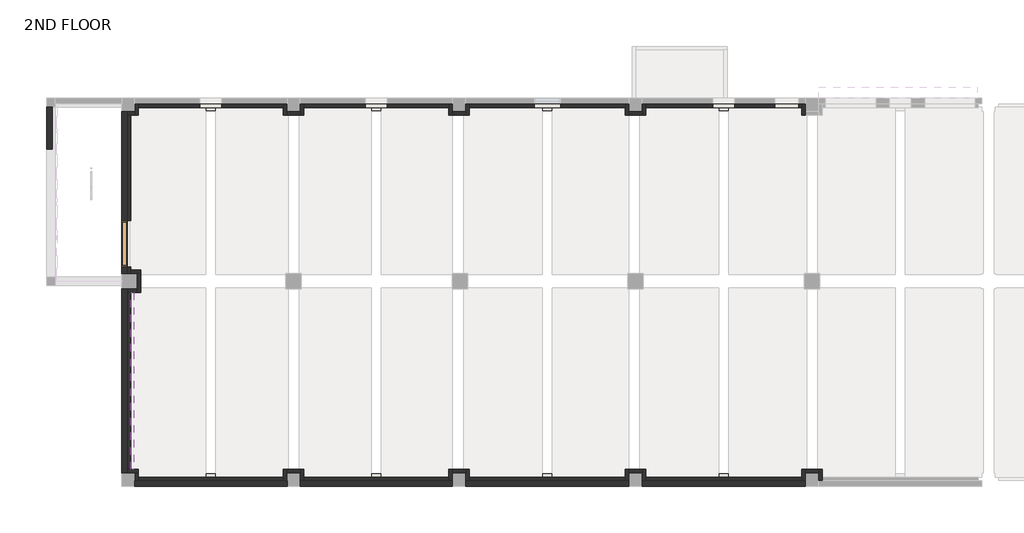
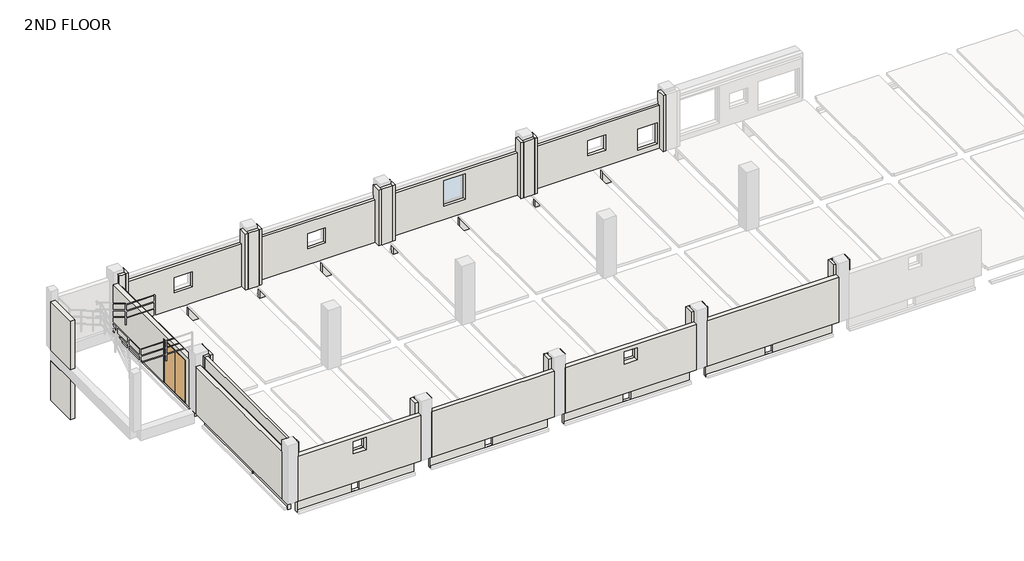
# One storey, part 1 of 7: 60 walls, 1 door.
"""IFC4 building model written with IfcOpenShell, lengths in millimetres."""

import ifcopenshell
import ifcopenshell.guid

model = None  # the IFC model being written
_history = None  # IfcOwnerHistory: only IFC2X3 demands one
_inside = {}  # id of a spatial element -> (the spatial element, [elements in it])
_under = {}  # id of a project, library or spatial element -> (it, [spatial elements below it])
_declared = {}  # id of a project -> (the project, [libraries it declares])
_typed = {}  # id of a type object -> (the type object, [elements of that type])
_made_of = {}  # id of a material, layer set ... -> (it, [elements and type objects made of it])


def new_model(schema):
    """Start an empty IFC model of exactly this schema.

    Asked for "IFC4X3", IfcOpenShell would pick the latest addendum, in which some entities
    have other attributes; the version numbers below select the first issue.
    IFC2X3 requires an IfcOwnerHistory on every rooted entity: one is made here for all.
    """
    global model, _history
    if schema == "IFC4X3":
        model = ifcopenshell.file(schema_version=(4, 3, 0, 0))
    else:
        model = ifcopenshell.file(schema=schema)
    _inside.clear()
    _under.clear()
    _declared.clear()
    _typed.clear()
    _made_of.clear()
    _history = None
    if model.schema == "IFC2X3":
        org = make("IfcOrganization", Name="unknown")
        user = make(
            "IfcPersonAndOrganization",
            ThePerson=make("IfcPerson", FamilyName="unknown"),
            TheOrganization=org,
        )
        app = make(
            "IfcApplication",
            ApplicationDeveloper=org,
            Version="unknown",
            ApplicationFullName="unknown",
            ApplicationIdentifier="unknown",
        )
        _history = make(
            "IfcOwnerHistory",
            OwningUser=user,
            OwningApplication=app,
            ChangeAction="ADDED",
            CreationDate=0,
        )
    return model


def make(cls, **values):
    """One entity of the class cls with the attributes given. An attribute that is None is left unset."""
    return model.create_entity(
        cls, **{name: value for name, value in values.items() if value is not None}
    )


def rooted(cls, **values):
    """An entity with a GlobalId (a new one), such as an element, a storey or a relation."""
    return make(cls, GlobalId=ifcopenshell.guid.new(), OwnerHistory=_history, **values)


def si_unit(unit_type, name, prefix=None):
    """IfcSIUnit, for example si_unit("LENGTHUNIT", "METRE", prefix="MILLI")."""
    return make("IfcSIUnit", UnitType=unit_type, Prefix=prefix, Name=name)


def assignment(units):
    """IfcUnitAssignment: the units of a project."""
    return None if units is None else make("IfcUnitAssignment", Units=units)


def point(xyz):
    """IfcCartesianPoint."""
    return None if xyz is None else make("IfcCartesianPoint", Coordinates=xyz)


def direction(xyz):
    """IfcDirection."""
    return None if xyz is None else make("IfcDirection", DirectionRatios=xyz)


def frame(location, z_axis=None, x_axis=None):
    """IfcAxis2Placement3D, a coordinate frame: its origin and axes. An axis left out is left unset."""
    return make(
        "IfcAxis2Placement3D",
        Location=point(location),
        Axis=direction(z_axis),
        RefDirection=direction(x_axis),
    )


def origin():
    """The frame at (0, 0, 0) with its axes left unset."""
    return frame((0.0, 0.0, 0.0))


def place(relative_to, where):
    """IfcLocalPlacement: puts the frame where relative to a parent placement (None: the world)."""
    return make(
        "IfcLocalPlacement", PlacementRelTo=relative_to, RelativePlacement=where
    )


def context(
    kind, dimensions, precision=None, world=None, true_north=None, identifier=None
):
    """IfcGeometricRepresentationContext, for example the 3D "Model" context."""
    return make(
        "IfcGeometricRepresentationContext",
        ContextIdentifier=identifier,
        ContextType=kind,
        CoordinateSpaceDimension=dimensions,
        Precision=precision,
        WorldCoordinateSystem=world,
        TrueNorth=true_north,
    )


def project(units=None, contexts=None):
    """IfcProject with its units and contexts."""
    return rooted(
        "IfcProject",
        Name="project",
        RepresentationContexts=contexts,
        UnitsInContext=assignment(units),
    )


def spatial(cls, under=None, at=None, **own):
    """A site, building, storey or space (cls), placed at a placement, below another one or the project."""
    s = rooted(cls, ObjectPlacement=at, **own)
    if under is not None:
        _under.setdefault(under.id(), (under, []))[1].append(s)
    return s


def polyline(points):
    """IfcPolyline through the points."""
    return make("IfcPolyline", Points=[point(p) for p in points])


def outline(outer, holes=None, kind="AREA"):
    """IfcArbitraryClosedProfileDef: a profile drawn as a closed curve; with holes, ...WithVoids."""
    if holes is None:
        return make("IfcArbitraryClosedProfileDef", ProfileType=kind, OuterCurve=outer)
    return make(
        "IfcArbitraryProfileDefWithVoids",
        ProfileType=kind,
        OuterCurve=outer,
        InnerCurves=holes,
    )


def extrude(swept, where, along, depth):
    """IfcExtrudedAreaSolid: the profile swept, set in the frame where, extruded along a direction by depth."""
    return make(
        "IfcExtrudedAreaSolid",
        SweptArea=swept,
        Position=where,
        ExtrudedDirection=direction(along),
        Depth=depth,
    )


def faces_of(points, faces, orient=None, outer=None):
    """IfcFace entities. A face is a list of loops; a loop is a list of indices into points, from 0.

    orient and outer hold one flag for each loop. By default every Orientation is true, the
    first loop of a face is its IfcFaceOuterBound and the others are IfcFaceBound.
    """
    made = []
    for i, loops in enumerate(faces):
        bounds = []
        for j, loop in enumerate(loops):
            is_outer = j == 0 if outer is None else outer[i][j]
            bounds.append(
                make(
                    "IfcFaceOuterBound" if is_outer else "IfcFaceBound",
                    Bound=make("IfcPolyLoop", Polygon=[points[k] for k in loop]),
                    Orientation=True if orient is None else orient[i][j],
                )
            )
        made.append(make("IfcFace", Bounds=bounds))
    return made


def faceted_brep(points, faces, orient=None, outer=None, voids=None):
    """IfcFacetedBrep: a solid bounded by flat faces; with voids (closed shells), ...WithVoids."""
    shared = [point(p) for p in points]
    hull = make("IfcClosedShell", CfsFaces=faces_of(shared, faces, orient, outer))
    if voids is None:
        return make("IfcFacetedBrep", Outer=hull)
    return make(
        "IfcFacetedBrepWithVoids",
        Outer=hull,
        Voids=[
            make(cls, CfsFaces=faces_of(shared, fs, o, b)) for cls, fs, o, b in voids
        ],
    )


def shape(context_of_items, identifier, shape_type, items):
    """IfcShapeRepresentation: the items that make up one representation, for example the "Body"."""
    return make(
        "IfcShapeRepresentation",
        ContextOfItems=context_of_items,
        RepresentationIdentifier=identifier,
        RepresentationType=shape_type,
        Items=items,
    )


def source(mapping_origin, context_of_items, identifier, shape_type, items):
    """IfcRepresentationMap: a shape defined once, which mapped items show again and again."""
    return make(
        "IfcRepresentationMap",
        MappingOrigin=mapping_origin,
        MappedRepresentation=shape(context_of_items, identifier, shape_type, items),
    )


def transform(
    local_origin,
    x_axis=None,
    y_axis=None,
    z_axis=None,
    scale=None,
    scale2=None,
    scale3=None,
    uniform=True,
):
    """IfcCartesianTransformationOperator3D, or its non-uniform kind. x_axis, y_axis, z_axis: its Axis1, 2, 3."""
    if uniform:
        return make(
            "IfcCartesianTransformationOperator3D",
            Axis1=direction(x_axis),
            Axis2=direction(y_axis),
            LocalOrigin=point(local_origin),
            Scale=scale,
            Axis3=direction(z_axis),
        )
    return make(
        "IfcCartesianTransformationOperator3DnonUniform",
        Axis1=direction(x_axis),
        Axis2=direction(y_axis),
        LocalOrigin=point(local_origin),
        Scale=scale,
        Axis3=direction(z_axis),
        Scale2=scale2,
        Scale3=scale3,
    )


def mapped(mapping_source, mapping_target):
    """IfcMappedItem: shows the shape of a source again, moved by a transform."""
    return make(
        "IfcMappedItem", MappingSource=mapping_source, MappingTarget=mapping_target
    )


def made_of(thing, what):
    """Note that an element or type object is made of a material, layer set ...; save() writes the relation."""
    if what is not None:
        _made_of.setdefault(what.id(), (what, []))[1].append(thing)
    return thing


def element(
    cls,
    number,
    at=None,
    inside=None,
    cuts=None,
    type_object=None,
    material=None,
    context=None,
    identifier="Body",
    shape_type=None,
    held_by="IfcProductDefinitionShape",
    body=None,
    shapes=None,
    **own,
):
    """One element of the class cls, such as IfcWall. Its Tag is "e" and its number.

    at: its placement. inside: the storey or other place that contains it. cuts: it is an
    opening in that element (IfcRelVoidsElement). A single representation is given by context,
    identifier, shape_type and body (its items); several are given by shapes. held_by: the class
    of the entity that holds the representations. save() writes the other relations.
    """
    e = rooted(cls, Tag="e%d" % number, ObjectPlacement=at, **own)
    if body is not None:
        shapes = [shape(context, identifier, shape_type, body)]
    if shapes is not None:
        e.Representation = make(held_by, Representations=shapes)
    if inside is not None:
        _inside.setdefault(inside.id(), (inside, []))[1].append(e)
    if cuts is not None:
        rooted(
            "IfcRelVoidsElement", RelatingBuildingElement=cuts, RelatedOpeningElement=e
        )
    if type_object is not None:
        _typed.setdefault(type_object.id(), (type_object, []))[1].append(e)
    return made_of(e, material)


def aggregate(whole, parts):
    """IfcRelAggregates: a whole, such as a stair, and the parts it consists of."""
    return rooted("IfcRelAggregates", RelatingObject=whole, RelatedObjects=parts)


def save(model, path):
    """Write the relations noted so far, then the file.

    IfcRelAggregates (storeys below a building ...), IfcRelContainedInSpatialStructure (elements
    in a storey), IfcRelDefinesByType, IfcRelAssociatesMaterial and IfcRelDeclares: one each for
    every whole, place, type object, material and project.
    """
    for whole, parts in _under.values():
        aggregate(whole, parts)
    for where, things in _inside.values():
        rooted(
            "IfcRelContainedInSpatialStructure",
            RelatedElements=things,
            RelatingStructure=where,
        )
    for kind, things in _typed.values():
        rooted("IfcRelDefinesByType", RelatedObjects=things, RelatingType=kind)
    for what, things in _made_of.values():
        rooted("IfcRelAssociatesMaterial", RelatedObjects=things, RelatingMaterial=what)
    for by, libraries in _declared.values():
        rooted("IfcRelDeclares", RelatingContext=by, RelatedDefinitions=libraries)
    model.write(path)


def double_door_steel_c24d22a6(model_context):
    return source(origin(), model_context, "Body", "SolidModel", [
        faceted_brep([(-1035.0, -125.0, 2565.0), (-1035.0, 125.0, 2565.0), (-1035.0, 125.0, 0.0), (-1035.0, -125.0, 0.0), (1035.0, 125.0, 0.0), (1035.0, 125.0, 2565.0), (1005.0, 125.0, 2535.0), (-1005.0, 125.0, 2535.0), (-1005.0, 125.0, 30.0), (1005.0, 125.0, 30.0), (1035.0, -125.0, 0.0), (1035.0, -125.0, 2565.0), (1005.0, -125.0, 30.0), (-1005.0, -125.0, 30.0), (-1005.0, -125.0, 2535.0), (1005.0, -125.0, 2535.0), (-1005.0, -85.0, 2535.0), (-1005.0, -85.0, 30.0), (1005.0, -85.0, 30.0), (1005.0, -85.0, 2535.0), (985.0, -85.0, 2515.0), (985.0, -85.0, 50.0), (-985.0, -85.0, 50.0), (-985.0, -85.0, 2515.0), (-985.0, 85.0, 2515.0), (-985.0, 85.0, 50.0), (985.0, 85.0, 50.0), (1005.0, 85.0, 30.0), (-1005.0, 85.0, 30.0), (-1005.0, 85.0, 2535.0), (1005.0, 85.0, 2535.0), (985.0, 85.0, 2515.0)], [[[0, 1, 2, 3]], [[4, 2, 1, 5], [6, 7, 8, 9]], [[3, 2, 4, 10]], [[11, 0, 3, 10], [12, 13, 14, 15]], [[16, 14, 13, 17]], [[17, 13, 12, 18]], [[16, 17, 18, 19], [20, 21, 22, 23]], [[24, 23, 22, 25]], [[25, 22, 21, 26]], [[27, 28, 29, 30], [31, 24, 25, 26]], [[7, 29, 28, 8]], [[8, 28, 27, 9]], [[10, 4, 5, 11]], [[9, 27, 30, 6]], [[18, 12, 15, 19]], [[26, 21, 20, 31]], [[11, 5, 1, 0]], [[19, 15, 14, 16]], [[31, 20, 23, 24]], [[6, 30, 29, 7]]]),
        extrude(outline(polyline([(1005.0, 85.0), (0.0, 85.0), (0.0, 125.0), (1005.0, 125.0), (1005.0, 85.0)])), frame((0.0, 0.0, 30.0), z_axis=(0.0, 0.0, 1.0), x_axis=(1.0, 0.0, 0.0)), (0.0, 0.0, 1.0), 2505.0),
        extrude(outline(polyline([(0.0, 85.0), (-1005.0, 85.0), (-1005.0, 125.0), (0.0, 125.0), (0.0, 85.0)])), frame((0.0, 0.0, 30.0), z_axis=(0.0, 0.0, 1.0), x_axis=(1.0, 0.0, 0.0)), (0.0, 0.0, 1.0), 2505.0),
    ])


model = new_model("IFC4")

# Units and contexts
model_context = context("Model", 3, world=origin())
ifc_project = project(units=[si_unit("LENGTHUNIT", "METRE", prefix="MILLI")], contexts=[model_context])

# Site, building, storey
site = spatial("IfcSite", under=ifc_project)
building = spatial("IfcBuilding", under=site)
storey = spatial("IfcBuildingStorey", under=building, Name="2ND FLOOR", Elevation=10600.0)

# Door
placement = place(None, origin())
double_door_steel_shape = double_door_steel_c24d22a6(model_context)
element("IfcDoor", 1, ObjectType="Double Door_Steel : H_DR_AR B12_Door_Double_W2100xH2580_No FR_SD-5", at=placement, inside=storey, context=model_context, shape_type="MappedRepresentation", body=[
    mapped(double_door_steel_shape, transform((-175.0, -6300.0, 10600.0), x_axis=(0.0, 1.0, 0.0), y_axis=(-1.0, 0.0, 0.0), z_axis=(0.0, 0.0, 1.0))),
])

# Walls
element("IfcWall", 2, ObjectType="H_WA_AR B02_Ext Wall RC-AG_T250_W1", at=placement, inside=storey, context=model_context, shape_type="SweptSolid", body=[
    extrude(outline(polyline([(23300.0, -17050.0), (30700.0, -17050.0), (30700.0, -17300.0), (23300.0, -17300.0), (23300.0, -17050.0)])), frame((0.0, 0.0, 10600.0), z_axis=(0.0, 0.0, 1.0), x_axis=(1.0, 0.0, 0.0)), (0.0, 0.0, 1.0), 2700.0),
])
element("IfcWall", 3, ObjectType="H_WA_AR B02_Ext Wall RC-AG_T250_W1", at=placement, inside=storey, context=model_context, shape_type="SweptSolid", body=[
    extrude(outline(polyline([(10600.0, 22700.0), (13300.0, 22700.0), (13300.0, 15299.9999999), (10600.0, 15299.9999999), (10600.0, 22700.0)]), holes=[polyline([(13070.0, 19360.0), (12350.0, 19360.0), (12350.0, 18640.0), (13070.0, 18640.0), (13070.0, 19360.0)])]), frame((0.0, -17300.0, 0.0), z_axis=(0.0, 1.0, 0.0), x_axis=(0.0, 0.0, 1.0)), (0.0, 0.0, 1.0), 250.0),
])
element("IfcWall", 4, ObjectType="H_WA_AR B02_Ext Wall RC-AG_T250_W1", at=placement, inside=storey, context=model_context, shape_type="SweptSolid", body=[
    extrude(outline(polyline([(7800.0, -17050.0), (14700.0, -17050.0), (14700.0, -17300.0), (7800.0, -17300.0), (7800.0, -17050.0)])), frame((0.0, 0.0, 10600.0), z_axis=(0.0, 0.0, 1.0), x_axis=(1.0, 0.0, 0.0)), (0.0, 0.0, 1.0), 2700.0),
])
element("IfcWall", 5, ObjectType="H_WA_AR B02_Ext Wall RC-AG_T250_W1", at=placement, inside=storey, context=model_context, shape_type="SweptSolid", body=[
    extrude(outline(polyline([(10600.0, 7200.0), (13300.0, 7200.0), (13300.0, 300.0), (10600.0, 300.0), (10600.0, 7200.0)]), holes=[polyline([(13070.0, 4110.0), (12350.0, 4110.0), (12350.0, 3390.0), (13070.0, 3390.0), (13070.0, 4110.0)])]), frame((0.0, -17300.0, 0.0), z_axis=(0.0, 1.0, 0.0), x_axis=(0.0, 0.0, 1.0)), (0.0, 0.0, 1.0), 250.0),
])
element("IfcWall", 6, ObjectType="H_WA_AR B02_Ext Wall RC-AG_T250_W1", at=placement, inside=storey, context=model_context, shape_type="SweptSolid", body=[
    extrude(outline(polyline([(-50.0, -8350.0), (-50.0, -16700.0), (-300.0, -16700.0), (-300.0, -8350.0), (-50.0, -8350.0)])), frame((0.0, 0.0, 10600.0), z_axis=(0.0, 0.0, 1.0), x_axis=(1.0, 0.0, 0.0)), (0.0, 0.0, 1.0), 2800.0),
])
element("IfcWall", 7, ObjectType="H_WA_AR B02_Ext Wall RC-AG_T250_W1", at=placement, inside=storey, context=model_context, shape_type="SweptSolid", body=[
    extrude(outline(polyline([(-300.0, 13400.0), (-300.0, 10600.0), (-5250.0, 10600.0), (-5250.0, 13180.0), (-7350.0, 13180.0), (-7350.0, 10600.0), (-7650.0, 10600.0), (-7650.0, 13400.0), (-300.0, 13400.0)])), frame((-300.0, 0.0, 0.0), z_axis=(1.0, 0.0, 0.0), x_axis=(0.0, 1.0, 0.0)), (0.0, 0.0, 1.0), 250.0),
])
element("IfcWall", 8, ObjectType="H_WA_AR B02_Ext Wall RC-AG_T250_W1", at=placement, inside=storey, context=model_context, shape_type="SweptSolid", body=[
    extrude(outline(polyline([(-3450.0, -100.0), (-3450.0, -2000.0), (-3700.0, -2000.0), (-3700.0, -100.0), (-3450.0, -100.0)])), frame((0.0, 0.0, 7590.0), z_axis=(0.0, 0.0, 1.0), x_axis=(1.0, 0.0, 0.0)), (0.0, 0.0, 1.0), 2360.0),
])
element("IfcWall", 9, ObjectType="H_WA_AR B02_Ext Wall RC-AG_T250_W1", at=placement, inside=storey, context=model_context, shape_type="Brep", body=[
    faceted_brep([(-3450.0, -2000.0, 10550.0), (-3450.0, -100.0, 10550.0), (-3450.0, -100.0, 13450.0), (-3450.0, -2000.0, 13450.0), (-3700.0, -2000.0, 10550.0), (-3700.0, -2000.0, 13450.0), (-3700.0, -100.0, 13450.0), (-3700.0, -100.0, 10600.0), (-3700.0, -100.0, 10550.0)], [[[0, 1, 2, 3]], [[4, 5, 6, 7, 8]], [[1, 0, 4, 8]], [[2, 1, 8, 7, 6]], [[3, 2, 6, 5]], [[0, 3, 5, 4]]]),
])
element("IfcWall", 10, ObjectType="H_WA_AR B02_Ext Wall DY-IN_T154", at=placement, inside=storey, context=model_context, shape_type="Brep", body=[
    faceted_brep([(464.0, -464.0, 10600.0), (464.0, -114.0, 10600.0), (464.0, 40.0, 10600.0), (464.0, 40.0, 13155.0), (464.0, 40.0, 13920.0), (464.0, -110.0, 13920.0), (464.0, -264.0, 13920.0), (464.0, -464.0, 13920.0), (310.0, -464.0, 10600.0), (310.0, -464.0, 13920.0), (310.0, -310.0, 13920.0), (310.0, 40.0, 13920.0), (310.0, 40.0, 10600.0), (310.0, -310.0, 10600.0)], [[[0, 1, 2, 3, 4, 5, 6, 7]], [[8, 9, 10, 11, 12, 13]], [[2, 1, 0, 8, 13, 12]], [[7, 6, 5, 4, 11, 10, 9]], [[4, 3, 2, 12, 11]], [[0, 7, 9, 8]]]),
])
element("IfcWall", 11, ObjectType="H_WA_AR B02_Ext Wall DY-IN_T154", at=placement, inside=storey, context=model_context, shape_type="SweptSolid", body=[
    extrude(outline(polyline([(10600.0, 464.0), (10600.0, 7036.0), (13136.0, 7036.0), (13136.0, 464.0), (10600.0, 464.0)]), holes=[polyline([(11550.0, 3250.0), (12450.0, 3250.0), (12450.0, 4250.0), (11550.0, 4250.0), (11550.0, 3250.0)])]), frame((0.0, -114.0, 0.0), z_axis=(0.0, 1.0, 0.0), x_axis=(0.0, 0.0, 1.0)), (0.0, 0.0, 1.0), 154.0),
])
element("IfcWall", 12, ObjectType="H_WA_AR B02_Ext Wall DY-IN_T154", at=placement, inside=storey, context=model_context, shape_type="Brep", body=[
    faceted_brep([(-40.0, -7640.0, 10600.0), (-40.0, -7640.0, 13255.0), (-40.0, -7486.0, 13255.0), (-40.0, -7486.0, 13236.0), (-40.0, -464.0, 13236.0), (-40.0, -464.0, 10600.0), (-40.0, -5250.0, 10600.0), (-40.0, -5250.0, 13180.0), (-40.0, -7350.0, 13180.0), (-40.0, -7350.0, 10600.0), (114.0, -7640.0, 13255.0), (114.0, -7640.0, 10600.0), (114.0, -7486.0, 10600.0), (114.0, -7350.0, 10600.0), (114.0, -7350.0, 13180.0), (114.0, -5250.0, 13180.0), (114.0, -5250.0, 10600.0), (114.0, -464.0, 10600.0), (114.0, -464.0, 13236.0), (114.0, -7486.0, 13236.0), (114.0, -7486.0, 13255.0), (110.0, -7486.0, 13255.0)], [[[0, 1, 2, 3, 4, 5, 6, 7, 8, 9]], [[10, 11, 12, 13, 14, 15, 16, 17, 18, 19, 20]], [[5, 17, 16, 6]], [[11, 0, 9, 13, 12]], [[1, 10, 20, 21, 2]], [[17, 5, 4, 18]], [[1, 0, 11, 10]], [[3, 19, 18, 4]], [[19, 3, 2, 21, 20]], [[15, 7, 6, 16]], [[7, 15, 14, 8]], [[8, 14, 13, 9]]]),
])
element("IfcWall", 13, ObjectType="H_WA_AR B02_Ext Wall DY-IN_T154", at=placement, inside=storey, context=model_context, shape_type="Brep", body=[
    faceted_brep([(310.0, -310.0, 10600.0), (-40.0, -310.0, 10600.0), (-40.0, -310.0, 13920.0), (310.0, -310.0, 13920.0), (310.0, -464.0, 10600.0), (310.0, -464.0, 13920.0), (264.0, -464.0, 13920.0), (110.0, -464.0, 13920.0), (-40.0, -464.0, 13920.0), (-40.0, -464.0, 13236.0), (-40.0, -464.0, 10600.0), (114.0, -464.0, 10600.0)], [[[0, 1, 2, 3]], [[4, 5, 6, 7, 8, 9, 10, 11]], [[1, 0, 4, 11, 10]], [[3, 2, 8, 7, 6, 5]], [[0, 3, 5, 4]], [[2, 1, 10, 9, 8]]]),
])
element("IfcWall", 14, ObjectType="H_WA_AR B02_Ext Wall DY-IN_T154", at=placement, inside=storey, context=model_context, shape_type="Brep", body=[
    faceted_brep([(114.0, -7640.0, 10600.0), (410.0, -7640.0, 10600.0), (564.0, -7640.0, 10600.0), (564.0, -7640.0, 13920.0), (410.0, -7640.0, 13920.0), (114.0, -7640.0, 13920.0), (114.0, -7640.0, 13255.0), (114.0, -7486.0, 10600.0), (114.0, -7486.0, 13236.0), (114.0, -7486.0, 13255.0), (114.0, -7486.0, 13920.0), (264.0, -7486.0, 13920.0), (564.0, -7486.0, 13920.0), (564.0, -7486.0, 10600.0)], [[[0, 1, 2, 3, 4, 5, 6]], [[7, 8, 9, 10, 11, 12, 13]], [[2, 1, 0, 7, 13]], [[5, 4, 3, 12, 11, 10]], [[3, 2, 13, 12]], [[0, 6, 5, 10, 9, 8, 7]]]),
])
element("IfcWall", 15, ObjectType="H_WA_AR B02_Ext Wall DY-IN_T154", at=placement, inside=storey, context=model_context, shape_type="Brep", body=[
    faceted_brep([(410.0, -7640.0, 10600.0), (410.0, -8360.0, 10600.0), (410.0, -8514.0, 10600.0), (410.0, -8514.0, 13920.0), (410.0, -8360.0, 13920.0), (410.0, -7640.0, 13920.0), (564.0, -7640.0, 10600.0), (564.0, -7640.0, 13920.0), (564.0, -8514.0, 13920.0), (564.0, -8514.0, 10600.0)], [[[0, 1, 2, 3, 4, 5]], [[6, 7, 8, 9]], [[2, 1, 0, 6, 9]], [[5, 4, 3, 8, 7]], [[0, 5, 7, 6]], [[3, 2, 9, 8]]]),
])
element("IfcWall", 16, ObjectType="H_WA_AR B02_Ext Wall DY-IN_T154", at=placement, inside=storey, context=model_context, shape_type="Brep", body=[
    faceted_brep([(410.0, -8360.0, 10600.0), (-40.0, -8360.0, 10600.0), (-40.0, -8360.0, 13255.0), (110.0, -8360.0, 13255.0), (110.0, -8360.0, 13920.0), (410.0, -8360.0, 13920.0), (410.0, -8514.0, 10600.0), (410.0, -8514.0, 13920.0), (264.0, -8514.0, 13920.0), (110.0, -8514.0, 13920.0), (110.0, -8514.0, 13255.0), (-40.0, -8514.0, 13255.0), (-40.0, -8514.0, 10600.0), (114.0, -8514.0, 10600.0)], [[[0, 1, 2, 3, 4, 5]], [[6, 7, 8, 9, 10, 11, 12, 13]], [[1, 0, 6, 13, 12]], [[5, 4, 9, 8, 7]], [[0, 5, 7, 6]], [[10, 3, 2, 11]], [[2, 1, 12, 11]], [[4, 3, 10, 9]]]),
])
element("IfcWall", 17, ObjectType="H_WA_AR B02_Ext Wall DY-IN_T154", at=placement, inside=storey, context=model_context, shape_type="SweptSolid", body=[
    extrude(outline(polyline([(-40.0, -16536.0), (-40.0, -8514.0), (114.0, -8514.0), (114.0, -16536.0), (-40.0, -16536.0)])), frame((0.0, 0.0, 10600.0), z_axis=(0.0, 0.0, 1.0), x_axis=(1.0, 0.0, 0.0)), (0.0, 0.0, 1.0), 2636.0),
])
element("IfcWall", 18, ObjectType="H_WA_AR B02_Ext Wall DY-IN_T154", at=placement, inside=storey, context=model_context, shape_type="Brep", body=[
    faceted_brep([(-40.0, -16690.0, 10600.0), (310.0, -16690.0, 10600.0), (464.0, -16690.0, 10600.0), (464.0, -16690.0, 13920.0), (310.0, -16690.0, 13920.0), (110.0, -16690.0, 13920.0), (110.0, -16690.0, 13255.0), (-40.0, -16690.0, 13255.0), (-40.0, -16536.0, 10600.0), (-40.0, -16536.0, 13236.0), (-40.0, -16536.0, 13255.0), (110.0, -16536.0, 13255.0), (110.0, -16536.0, 13920.0), (264.0, -16536.0, 13920.0), (464.0, -16536.0, 13920.0), (464.0, -16536.0, 10600.0), (114.0, -16536.0, 10600.0)], [[[0, 1, 2, 3, 4, 5, 6, 7]], [[8, 9, 10, 11, 12, 13, 14, 15, 16]], [[2, 1, 0, 8, 16, 15]], [[5, 4, 3, 14, 13, 12]], [[3, 2, 15, 14]], [[6, 11, 10, 7]], [[0, 7, 10, 9, 8]], [[6, 5, 12, 11]]]),
])
element("IfcWall", 19, ObjectType="H_WA_AR B02_Ext Wall DY-IN_T154", at=placement, inside=storey, context=model_context, shape_type="Brep", body=[
    faceted_brep([(310.0, -16690.0, 10600.0), (310.0, -17040.0, 10600.0), (310.0, -17040.0, 13920.0), (310.0, -16690.0, 13920.0), (464.0, -16690.0, 10600.0), (464.0, -16690.0, 13920.0), (464.0, -16736.0, 13920.0), (464.0, -16890.0, 13920.0), (464.0, -17040.0, 13920.0), (464.0, -17040.0, 13155.0), (464.0, -17040.0, 10600.0), (464.0, -16886.0, 10600.0)], [[[0, 1, 2, 3]], [[4, 5, 6, 7, 8, 9, 10, 11]], [[1, 0, 4, 11, 10]], [[3, 2, 8, 7, 6, 5]], [[0, 3, 5, 4]], [[2, 1, 10, 9, 8]]]),
])
element("IfcWall", 20, ObjectType="H_WA_AR B02_Ext Wall DY-IN_T154", at=placement, inside=storey, context=model_context, shape_type="SweptSolid", body=[
    extrude(outline(polyline([(10600.0, 464.0), (10600.0, 7036.0), (13136.0, 7036.0), (13136.0, 464.0), (10600.0, 464.0)]), holes=[polyline([(13070.0, 4110.0), (12350.0, 4110.0), (12350.0, 3390.0), (13070.0, 3390.0), (13070.0, 4110.0)])]), frame((0.0, -17040.0, 0.0), z_axis=(0.0, 1.0, 0.0), x_axis=(0.0, 0.0, 1.0)), (0.0, 0.0, 1.0), 154.0),
])
element("IfcWall", 21, ObjectType="H_WA_AR B02_Ext Wall DY-IN_T154", at=placement, inside=storey, context=model_context, shape_type="Brep", body=[
    faceted_brep([(7190.0, -17040.0, 10600.0), (7190.0, -16690.0, 10600.0), (7190.0, -16536.0, 10600.0), (7190.0, -16536.0, 13920.0), (7190.0, -16690.0, 13920.0), (7190.0, -17040.0, 13920.0), (7036.0, -17040.0, 10600.0), (7036.0, -17040.0, 13155.0), (7036.0, -17040.0, 13920.0), (7036.0, -16890.0, 13920.0), (7036.0, -16736.0, 13920.0), (7036.0, -16536.0, 13920.0), (7036.0, -16536.0, 10600.0), (7036.0, -16886.0, 10600.0)], [[[0, 1, 2, 3, 4, 5]], [[6, 7, 8, 9, 10, 11, 12, 13]], [[2, 1, 0, 6, 13, 12]], [[5, 4, 3, 11, 10, 9, 8]], [[3, 2, 12, 11]], [[0, 5, 8, 7, 6]]]),
])
element("IfcWall", 22, ObjectType="H_WA_AR B02_Ext Wall DY-IN_T154", at=placement, inside=storey, context=model_context, shape_type="SweptSolid", body=[
    extrude(outline(polyline([(7810.0, -16690.0), (7190.0, -16690.0), (7190.0, -16536.0), (7810.0, -16536.0), (7810.0, -16690.0)])), frame((0.0, 0.0, 10600.0), z_axis=(0.0, 0.0, 1.0), x_axis=(1.0, 0.0, 0.0)), (0.0, 0.0, 1.0), 3320.0),
])
element("IfcWall", 23, ObjectType="H_WA_AR B02_Ext Wall DY-IN_T154", at=placement, inside=storey, context=model_context, shape_type="Brep", body=[
    faceted_brep([(7810.0, -16536.0, 10600.0), (7810.0, -16690.0, 10600.0), (7810.0, -17040.0, 10600.0), (7810.0, -17040.0, 13920.0), (7810.0, -16690.0, 13920.0), (7810.0, -16536.0, 13920.0), (7964.0, -16536.0, 10600.0), (7964.0, -16536.0, 13920.0), (7964.0, -16736.0, 13920.0), (7964.0, -16890.0, 13920.0), (7964.0, -17040.0, 13920.0), (7964.0, -17040.0, 13155.0), (7964.0, -17040.0, 10600.0), (7964.0, -16886.0, 10600.0)], [[[0, 1, 2, 3, 4, 5]], [[6, 7, 8, 9, 10, 11, 12, 13]], [[2, 1, 0, 6, 13, 12]], [[5, 4, 3, 10, 9, 8, 7]], [[0, 5, 7, 6]], [[3, 2, 12, 11, 10]]]),
])
element("IfcWall", 24, ObjectType="H_WA_AR B02_Ext Wall DY-IN_T154", at=placement, inside=storey, context=model_context, shape_type="SweptSolid", body=[
    extrude(outline(polyline([(14536.0, -17040.0), (7964.0, -17040.0), (7964.0, -16886.0), (14536.0, -16886.0), (14536.0, -17040.0)])), frame((0.0, 0.0, 10600.0), z_axis=(0.0, 0.0, 1.0), x_axis=(1.0, 0.0, 0.0)), (0.0, 0.0, 1.0), 2536.0),
])
element("IfcWall", 25, ObjectType="H_WA_AR B02_Ext Wall DY-IN_T154", at=placement, inside=storey, context=model_context, shape_type="Brep", body=[
    faceted_brep([(14690.0, -17040.0, 10600.0), (14690.0, -16690.0, 10600.0), (14690.0, -16536.0, 10600.0), (14690.0, -16536.0, 13920.0), (14690.0, -16690.0, 13920.0), (14690.0, -17040.0, 13920.0), (14536.0, -17040.0, 10600.0), (14536.0, -17040.0, 13155.0), (14536.0, -17040.0, 13920.0), (14536.0, -16890.0, 13920.0), (14536.0, -16736.0, 13920.0), (14536.0, -16536.0, 13920.0), (14536.0, -16536.0, 10600.0), (14536.0, -16886.0, 10600.0)], [[[0, 1, 2, 3, 4, 5]], [[6, 7, 8, 9, 10, 11, 12, 13]], [[2, 1, 0, 6, 13, 12]], [[5, 4, 3, 11, 10, 9, 8]], [[3, 2, 12, 11]], [[0, 5, 8, 7, 6]]]),
])
element("IfcWall", 26, ObjectType="H_WA_AR B02_Ext Wall DY-IN_T154", at=placement, inside=storey, context=model_context, shape_type="SweptSolid", body=[
    extrude(outline(polyline([(15310.0, -16690.0), (14690.0, -16690.0), (14690.0, -16536.0), (15310.0, -16536.0), (15310.0, -16690.0)])), frame((0.0, 0.0, 10600.0), z_axis=(0.0, 0.0, 1.0), x_axis=(1.0, 0.0, 0.0)), (0.0, 0.0, 1.0), 3320.0),
])
element("IfcWall", 27, ObjectType="H_WA_AR B02_Ext Wall DY-IN_T154", at=placement, inside=storey, context=model_context, shape_type="Brep", body=[
    faceted_brep([(15310.0, -16536.0, 10600.0), (15310.0, -16690.0, 10600.0), (15310.0, -17040.0, 10600.0), (15310.0, -17040.0, 13920.0), (15310.0, -16690.0, 13920.0), (15310.0, -16536.0, 13920.0), (15464.0, -16536.0, 10600.0), (15464.0, -16536.0, 13920.0), (15464.0, -16736.0, 13920.0), (15464.0, -16890.0, 13920.0), (15464.0, -17040.0, 13920.0), (15464.0, -17040.0, 13155.0), (15464.0, -17040.0, 10600.0), (15464.0, -16886.0, 10600.0)], [[[0, 1, 2, 3, 4, 5]], [[6, 7, 8, 9, 10, 11, 12, 13]], [[2, 1, 0, 6, 13, 12]], [[5, 4, 3, 10, 9, 8, 7]], [[0, 5, 7, 6]], [[3, 2, 12, 11, 10]]]),
])
element("IfcWall", 28, ObjectType="H_WA_AR B02_Ext Wall DY-IN_T154", at=placement, inside=storey, context=model_context, shape_type="SweptSolid", body=[
    extrude(outline(polyline([(10600.0, 15464.0), (10600.0, 22536.0), (13136.0, 22536.0), (13136.0, 15464.0), (10600.0, 15464.0)]), holes=[polyline([(13070.0, 19360.0), (12350.0, 19360.0), (12350.0, 18640.0), (13070.0, 18640.0), (13070.0, 19360.0)])]), frame((0.0, -17040.0, 0.0), z_axis=(0.0, 1.0, 0.0), x_axis=(0.0, 0.0, 1.0)), (0.0, 0.0, 1.0), 154.0),
])
element("IfcWall", 29, ObjectType="H_WA_AR B02_Ext Wall DY-IN_T154", at=placement, inside=storey, context=model_context, shape_type="Brep", body=[
    faceted_brep([(22690.0, -17040.0, 10600.0), (22690.0, -16690.0, 10600.0), (22690.0, -16536.0, 10600.0), (22690.0, -16536.0, 13920.0), (22690.0, -16690.0, 13920.0), (22690.0, -17040.0, 13920.0), (22536.0, -17040.0, 10600.0), (22536.0, -17040.0, 13155.0), (22536.0, -17040.0, 13920.0), (22536.0, -16890.0, 13920.0), (22536.0, -16736.0, 13920.0), (22536.0, -16536.0, 13920.0), (22536.0, -16536.0, 10600.0), (22536.0, -16886.0, 10600.0)], [[[0, 1, 2, 3, 4, 5]], [[6, 7, 8, 9, 10, 11, 12, 13]], [[2, 1, 0, 6, 13, 12]], [[5, 4, 3, 11, 10, 9, 8]], [[0, 5, 8, 7, 6]], [[3, 2, 12, 11]]]),
])
element("IfcWall", 30, ObjectType="H_WA_AR B02_Ext Wall DY-IN_T154", at=placement, inside=storey, context=model_context, shape_type="SweptSolid", body=[
    extrude(outline(polyline([(23310.0, -16690.0), (22690.0, -16690.0), (22690.0, -16536.0), (23310.0, -16536.0), (23310.0, -16690.0)])), frame((0.0, 0.0, 10600.0), z_axis=(0.0, 0.0, 1.0), x_axis=(1.0, 0.0, 0.0)), (0.0, 0.0, 1.0), 3320.0),
])
element("IfcWall", 31, ObjectType="H_WA_AR B02_Ext Wall DY-IN_T154", at=placement, inside=storey, context=model_context, shape_type="Brep", body=[
    faceted_brep([(23310.0, -16536.0, 10600.0), (23310.0, -16690.0, 10600.0), (23310.0, -17040.0, 10600.0), (23310.0, -17040.0, 13920.0), (23310.0, -16690.0, 13920.0), (23310.0, -16536.0, 13920.0), (23464.0, -16536.0, 10600.0), (23464.0, -16536.0, 13920.0), (23464.0, -16736.0, 13920.0), (23464.0, -16890.0, 13920.0), (23464.0, -17040.0, 13920.0), (23464.0, -17040.0, 13155.0), (23464.0, -17040.0, 10600.0), (23464.0, -16886.0, 10600.0)], [[[0, 1, 2, 3, 4, 5]], [[6, 7, 8, 9, 10, 11, 12, 13]], [[2, 1, 0, 6, 13, 12]], [[5, 4, 3, 10, 9, 8, 7]], [[0, 5, 7, 6]], [[3, 2, 12, 11, 10]]]),
])
element("IfcWall", 32, ObjectType="H_WA_AR B02_Ext Wall DY-IN_T154", at=placement, inside=storey, context=model_context, shape_type="SweptSolid", body=[
    extrude(outline(polyline([(30536.0, -17040.0), (23464.0, -17040.0), (23464.0, -16886.0), (30536.0, -16886.0), (30536.0, -17040.0)])), frame((0.0, 0.0, 10600.0), z_axis=(0.0, 0.0, 1.0), x_axis=(1.0, 0.0, 0.0)), (0.0, 0.0, 1.0), 2536.0),
])
element("IfcWall", 33, ObjectType="H_WA_AR B02_Ext Wall DY-IN_T154", at=placement, inside=storey, context=model_context, shape_type="Brep", body=[
    faceted_brep([(30690.0, -17040.0, 10600.0), (30690.0, -16690.0, 10600.0), (30690.0, -16536.0, 10600.0), (30690.0, -16536.0, 13920.0), (30690.0, -16690.0, 13920.0), (30690.0, -17040.0, 13920.0), (30536.0, -17040.0, 10600.0), (30536.0, -17040.0, 13155.0), (30536.0, -17040.0, 13920.0), (30536.0, -16890.0, 13920.0), (30536.0, -16736.0, 13920.0), (30536.0, -16536.0, 13920.0), (30536.0, -16536.0, 10600.0), (30536.0, -16886.0, 10600.0)], [[[0, 1, 2, 3, 4, 5]], [[6, 7, 8, 9, 10, 11, 12, 13]], [[2, 1, 0, 6, 13, 12]], [[5, 4, 3, 11, 10, 9, 8]], [[3, 2, 12, 11]], [[0, 5, 8, 7, 6]]]),
])
element("IfcWall", 34, ObjectType="H_WA_AR B02_Ext Wall DY-IN_T154", at=placement, inside=storey, context=model_context, shape_type="SweptSolid", body=[
    extrude(outline(polyline([(31310.0, -16690.0), (30690.0, -16690.0), (30690.0, -16536.0), (31310.0, -16536.0), (31310.0, -16690.0)])), frame((0.0, 0.0, 10600.0), z_axis=(0.0, 0.0, 1.0), x_axis=(1.0, 0.0, 0.0)), (0.0, 0.0, 1.0), 3320.0),
])
element("IfcWall", 35, ObjectType="H_WA_AR B02_Ext Wall DY-IN_T154", at=placement, inside=storey, context=model_context, shape_type="Brep", body=[
    faceted_brep([(31310.0, -16536.0, 10600.0), (31310.0, -16690.0, 10600.0), (31310.0, -17040.0, 10600.0), (31310.0, -17040.0, 13920.0), (31310.0, -16690.0, 13920.0), (31310.0, -16536.0, 13920.0), (31464.0, -16536.0, 10600.0), (31464.0, -16536.0, 13920.0), (31464.0, -16736.0, 13920.0), (31464.0, -16890.0, 13920.0), (31464.0, -17040.0, 13920.0), (31464.0, -17040.0, 13155.0), (31464.0, -17040.0, 10600.0), (31464.0, -16886.0, 10600.0)], [[[0, 1, 2, 3, 4, 5]], [[6, 7, 8, 9, 10, 11, 12, 13]], [[2, 1, 0, 6, 13, 12]], [[5, 4, 3, 10, 9, 8, 7]], [[0, 5, 7, 6]], [[3, 2, 12, 11, 10]]]),
])
element("IfcWall", 36, ObjectType="H_WA_AR B02_Ext Wall DY-IN_T154", at=placement, inside=storey, context=model_context, shape_type="Brep", body=[
    faceted_brep([(7036.0, 40.0, 10600.0), (7036.0, -114.0, 10600.0), (7036.0, -464.0, 10600.0), (7036.0, -464.0, 13920.0), (7036.0, -264.0, 13920.0), (7036.0, -110.0, 13920.0), (7036.0, 40.0, 13920.0), (7036.0, 40.0, 13155.0), (7190.0, 40.0, 10600.0), (7190.0, 40.0, 13920.0), (7190.0, -310.0, 13920.0), (7190.0, -464.0, 13920.0), (7190.0, -464.0, 10600.0), (7190.0, -310.0, 10600.0)], [[[0, 1, 2, 3, 4, 5, 6, 7]], [[8, 9, 10, 11, 12, 13]], [[2, 1, 0, 8, 13, 12]], [[6, 5, 4, 3, 11, 10, 9]], [[3, 2, 12, 11]], [[0, 7, 6, 9, 8]]]),
])
element("IfcWall", 37, ObjectType="H_WA_AR B02_Ext Wall DY-IN_T154", at=placement, inside=storey, context=model_context, shape_type="SweptSolid", body=[
    extrude(outline(polyline([(7810.0, -464.0), (7190.0, -464.0), (7190.0, -310.0), (7810.0, -310.0), (7810.0, -464.0)])), frame((0.0, 0.0, 10600.0), z_axis=(0.0, 0.0, 1.0), x_axis=(1.0, 0.0, 0.0)), (0.0, 0.0, 1.0), 3320.0),
])
element("IfcWall", 38, ObjectType="H_WA_AR B02_Ext Wall DY-IN_T154", at=placement, inside=storey, context=model_context, shape_type="Brep", body=[
    faceted_brep([(7964.0, -464.0, 10600.0), (7964.0, -114.0, 10600.0), (7964.0, 40.0, 10600.0), (7964.0, 40.0, 13155.0), (7964.0, 40.0, 13920.0), (7964.0, -110.0, 13920.0), (7964.0, -264.0, 13920.0), (7964.0, -464.0, 13920.0), (7810.0, -464.0, 10600.0), (7810.0, -464.0, 13920.0), (7810.0, -310.0, 13920.0), (7810.0, 40.0, 13920.0), (7810.0, 40.0, 10600.0), (7810.0, -310.0, 10600.0)], [[[0, 1, 2, 3, 4, 5, 6, 7]], [[8, 9, 10, 11, 12, 13]], [[2, 1, 0, 8, 13, 12]], [[7, 6, 5, 4, 11, 10, 9]], [[0, 7, 9, 8]], [[4, 3, 2, 12, 11]]]),
])
element("IfcWall", 39, ObjectType="H_WA_AR B02_Ext Wall DY-IN_T154", at=placement, inside=storey, context=model_context, shape_type="SweptSolid", body=[
    extrude(outline(polyline([(10600.0, 7964.0), (10600.0, 14536.0), (13136.0, 14536.0), (13136.0, 7964.0), (10600.0, 7964.0)]), holes=[polyline([(11550.0, 10750.0), (12450.0, 10750.0), (12450.0, 11750.0), (11550.0, 11750.0), (11550.0, 10750.0)])]), frame((0.0, -114.0, 0.0), z_axis=(0.0, 1.0, 0.0), x_axis=(0.0, 0.0, 1.0)), (0.0, 0.0, 1.0), 154.0),
])
element("IfcWall", 40, ObjectType="H_WA_AR B02_Ext Wall DY-IN_T154", at=placement, inside=storey, context=model_context, shape_type="Brep", body=[
    faceted_brep([(14536.0, 40.0, 10600.0), (14536.0, -114.0, 10600.0), (14536.0, -464.0, 10600.0), (14536.0, -464.0, 13920.0), (14536.0, -264.0, 13920.0), (14536.0, -110.0, 13920.0), (14536.0, 40.0, 13920.0), (14536.0, 40.0, 13155.0), (14690.0, 40.0, 10600.0), (14690.0, 40.0, 13920.0), (14690.0, -310.0, 13920.0), (14690.0, -464.0, 13920.0), (14690.0, -464.0, 10600.0), (14690.0, -310.0, 10600.0)], [[[0, 1, 2, 3, 4, 5, 6, 7]], [[8, 9, 10, 11, 12, 13]], [[2, 1, 0, 8, 13, 12]], [[6, 5, 4, 3, 11, 10, 9]], [[3, 2, 12, 11]], [[0, 7, 6, 9, 8]]]),
])
element("IfcWall", 41, ObjectType="H_WA_AR B02_Ext Wall DY-IN_T154", at=placement, inside=storey, context=model_context, shape_type="SweptSolid", body=[
    extrude(outline(polyline([(15310.0, -464.0), (14690.0, -464.0), (14690.0, -310.0), (15310.0, -310.0), (15310.0, -464.0)])), frame((0.0, 0.0, 10600.0), z_axis=(0.0, 0.0, 1.0), x_axis=(1.0, 0.0, 0.0)), (0.0, 0.0, 1.0), 3320.0),
])
element("IfcWall", 42, ObjectType="H_WA_AR B02_Ext Wall DY-IN_T154", at=placement, inside=storey, context=model_context, shape_type="Brep", body=[
    faceted_brep([(15464.0, -464.0, 10600.0), (15464.0, -114.0, 10600.0), (15464.0, 40.0, 10600.0), (15464.0, 40.0, 13155.0), (15464.0, 40.0, 13920.0), (15464.0, -110.0, 13920.0), (15464.0, -264.0, 13920.0), (15464.0, -464.0, 13920.0), (15310.0, -464.0, 10600.0), (15310.0, -464.0, 13920.0), (15310.0, -310.0, 13920.0), (15310.0, 40.0, 13920.0), (15310.0, 40.0, 10600.0), (15310.0, -310.0, 10600.0)], [[[0, 1, 2, 3, 4, 5, 6, 7]], [[8, 9, 10, 11, 12, 13]], [[2, 1, 0, 8, 13, 12]], [[7, 6, 5, 4, 11, 10, 9]], [[0, 7, 9, 8]], [[4, 3, 2, 12, 11]]]),
])
element("IfcWall", 43, ObjectType="H_WA_AR B02_Ext Wall DY-IN_T154", at=placement, inside=storey, context=model_context, shape_type="SweptSolid", body=[
    extrude(outline(polyline([(10600.0, 15464.0), (10600.0, 22536.0), (13136.0, 22536.0), (13136.0, 15464.0), (10600.0, 15464.0)]), holes=[polyline([(12900.0, 19599.9999999), (11400.0, 19599.9999999), (11400.0, 18399.9999999), (12900.0, 18399.9999999), (12900.0, 19599.9999999)])]), frame((0.0, -114.0, 0.0), z_axis=(0.0, 1.0, 0.0), x_axis=(0.0, 0.0, 1.0)), (0.0, 0.0, 1.0), 154.0),
])
element("IfcWall", 44, ObjectType="H_WA_AR B02_Ext Wall DY-IN_T154", at=placement, inside=storey, context=model_context, shape_type="Brep", body=[
    faceted_brep([(22536.0, 40.0, 10600.0), (22536.0, -114.0, 10600.0), (22536.0, -464.0, 10600.0), (22536.0, -464.0, 13920.0), (22536.0, -264.0, 13920.0), (22536.0, -110.0, 13920.0), (22536.0, 40.0, 13920.0), (22536.0, 40.0, 13155.0), (22690.0, 40.0, 10600.0), (22690.0, 40.0, 13920.0), (22690.0, -310.0, 13920.0), (22690.0, -464.0, 13920.0), (22690.0, -464.0, 10600.0), (22690.0, -310.0, 10600.0)], [[[0, 1, 2, 3, 4, 5, 6, 7]], [[8, 9, 10, 11, 12, 13]], [[2, 1, 0, 8, 13, 12]], [[6, 5, 4, 3, 11, 10, 9]], [[0, 7, 6, 9, 8]], [[3, 2, 12, 11]]]),
])
element("IfcWall", 45, ObjectType="H_WA_AR B02_Ext Wall DY-IN_T154", at=placement, inside=storey, context=model_context, shape_type="SweptSolid", body=[
    extrude(outline(polyline([(23310.0, -464.0), (22690.0, -464.0), (22690.0, -310.0), (23310.0, -310.0), (23310.0, -464.0)])), frame((0.0, 0.0, 10600.0), z_axis=(0.0, 0.0, 1.0), x_axis=(1.0, 0.0, 0.0)), (0.0, 0.0, 1.0), 3320.0),
])
element("IfcWall", 46, ObjectType="H_WA_AR B02_Ext Wall DY-IN_T154", at=placement, inside=storey, context=model_context, shape_type="Brep", body=[
    faceted_brep([(23464.0, -464.0, 10600.0), (23464.0, -114.0, 10600.0), (23464.0, 40.0, 10600.0), (23464.0, 40.0, 13155.0), (23464.0, 40.0, 13920.0), (23464.0, -110.0, 13920.0), (23464.0, -264.0, 13920.0), (23464.0, -464.0, 13920.0), (23310.0, -464.0, 10600.0), (23310.0, -464.0, 13920.0), (23310.0, -310.0, 13920.0), (23310.0, 40.0, 13920.0), (23310.0, 40.0, 10600.0), (23310.0, -310.0, 10600.0)], [[[0, 1, 2, 3, 4, 5, 6, 7]], [[8, 9, 10, 11, 12, 13]], [[2, 1, 0, 8, 13, 12]], [[7, 6, 5, 4, 11, 10, 9]], [[0, 7, 9, 8]], [[4, 3, 2, 12, 11]]]),
])
element("IfcWall", 47, ObjectType="H_WA_AR B02_Ext Wall DY-IN_T154", at=placement, inside=storey, context=model_context, shape_type="SweptSolid", body=[
    extrude(outline(polyline([(10600.0, 23464.0), (10600.0, 30536.0), (13136.0, 30536.0), (13136.0, 23464.0), (10600.0, 23464.0)]), holes=[polyline([(10900.0, 29300.0), (12150.0, 29300.0), (12150.0, 30400.0), (10900.0, 30400.0), (10900.0, 29300.0)]), polyline([(11550.0, 26500.0), (12450.0, 26500.0), (12450.0, 27500.0), (11550.0, 27500.0), (11550.0, 26500.0)])]), frame((0.0, -114.0, 0.0), z_axis=(0.0, 1.0, 0.0), x_axis=(0.0, 0.0, 1.0)), (0.0, 0.0, 1.0), 154.0),
])
element("IfcWall", 48, ObjectType="H_WA_AR B02_Ext Wall DY-IN_T154", at=placement, inside=storey, context=model_context, shape_type="Brep", body=[
    faceted_brep([(30536.0, 40.0, 10600.0), (30536.0, -114.0, 10600.0), (30536.0, -464.0, 10600.0), (30536.0, -464.0, 13920.0), (30536.0, -264.0, 13920.0), (30536.0, -110.0, 13920.0), (30536.0, 40.0, 13920.0), (30536.0, 40.0, 13155.0), (30690.0, 40.0, 10600.0), (30690.0, 40.0, 13920.0), (30690.0, -310.0, 13920.0), (30690.0, -464.0, 13920.0), (30690.0, -464.0, 10600.0), (30690.0, -310.0, 10600.0)], [[[0, 1, 2, 3, 4, 5, 6, 7]], [[8, 9, 10, 11, 12, 13]], [[2, 1, 0, 8, 13, 12]], [[6, 5, 4, 3, 11, 10, 9]], [[3, 2, 12, 11]], [[0, 7, 6, 9, 8]]]),
])
element("IfcWall", 49, ObjectType="H_WA_AR B02_Ext Wall DY-IN_T154", at=placement, inside=storey, context=model_context, shape_type="Brep", body=[
    faceted_brep([(110.0, -8514.0, 13255.0), (110.0, -16536.0, 13255.0), (110.0, -16536.0, 13390.0), (110.0, -16536.0, 13920.0), (110.0, -8514.0, 13920.0), (110.0, -8514.0, 13390.0), (264.0, -8514.0, 13255.0), (264.0, -8514.0, 13920.0), (264.0, -16536.0, 13920.0), (264.0, -16536.0, 13255.0)], [[[0, 1, 2, 3, 4, 5]], [[6, 7, 8, 9]], [[1, 0, 6, 9]], [[4, 3, 8, 7]], [[0, 5, 4, 7, 6]], [[3, 2, 1, 9, 8]]]),
])
element("IfcWall", 50, ObjectType="H_WA_AR B02_Ext Wall DY-IN_T154", at=placement, inside=storey, context=model_context, shape_type="Brep", body=[
    faceted_brep([(264.0, -16613.0, 9755.0), (264.0, -16536.0, 9755.0), (264.0, -13264.0, 9755.0), (264.0, -13264.0, 10450.0), (264.0, -16613.0, 10450.0), (110.0, -16613.0, 9755.0), (110.0, -16613.0, 10450.0), (110.0, -13264.0, 10450.0), (110.0, -13264.0, 9890.0), (110.0, -13264.0, 9755.0), (110.0, -16536.0, 9755.0), (114.0, -13264.0, 10450.0)], [[[0, 1, 2, 3, 4]], [[5, 6, 7, 8, 9, 10]], [[2, 1, 0, 5, 10, 9]], [[4, 3, 11, 7, 6]], [[0, 4, 6, 5]], [[3, 2, 9, 8, 7, 11]]]),
])
element("IfcWall", 51, ObjectType="H_WA_AR B02_Ext Wall DY-IN_T154", at=placement, inside=storey, context=model_context, shape_type="Brep", body=[
    faceted_brep([(264.0, -13136.0, 9755.0), (264.0, -8514.0, 9755.0), (264.0, -8514.0, 10450.0), (264.0, -13136.0, 10450.0), (110.0, -13136.0, 9755.0), (110.0, -13136.0, 9890.0), (110.0, -13136.0, 10450.0), (110.0, -8514.0, 10450.0), (110.0, -8514.0, 10420.0), (110.0, -8514.0, 9890.0), (110.0, -8514.0, 9755.0), (114.0, -13136.0, 10450.0)], [[[0, 1, 2, 3]], [[4, 5, 6, 7, 8, 9, 10]], [[1, 0, 4, 10]], [[3, 2, 7, 6, 11]], [[0, 3, 11, 6, 5, 4]], [[2, 1, 10, 9, 8, 7]]]),
])
element("IfcWall", 52, ObjectType="H_WA_AR B02_Ext Wall DY-IN_T154", at=placement, inside=storey, context=model_context, shape_type="Brep", body=[
    faceted_brep([(464.0, -16890.0, 9655.0), (7036.0, -16890.0, 9655.0), (7036.0, -16890.0, 9790.0), (7036.0, -16890.0, 10450.0), (3975.0, -16890.0, 10450.0), (3975.0, -16890.0, 9800.0), (3525.0, -16890.0, 9800.0), (3525.0, -16890.0, 10450.0), (464.0, -16890.0, 10450.0), (464.0, -16890.0, 9790.0), (7036.0, -16736.0, 9655.0), (464.0, -16736.0, 9655.0), (464.0, -16736.0, 10450.0), (3525.0, -16736.0, 10450.0), (3525.0, -16736.0, 9800.0), (3975.0, -16736.0, 9800.0), (3975.0, -16736.0, 10450.0), (7036.0, -16736.0, 10450.0)], [[[0, 1, 2, 3, 4, 5, 6, 7, 8, 9]], [[10, 11, 12, 13, 14, 15, 16, 17]], [[1, 0, 11, 10]], [[12, 8, 7, 13]], [[3, 17, 16, 4]], [[0, 9, 8, 12, 11]], [[3, 2, 1, 10, 17]], [[6, 14, 13, 7]], [[14, 6, 5, 15]], [[15, 5, 4, 16]]]),
])
element("IfcWall", 53, ObjectType="H_WA_AR B02_Ext Wall DY-IN_T154", at=placement, inside=storey, context=model_context, shape_type="Brep", body=[
    faceted_brep([(7964.0, -16890.0, 9655.0), (14536.0, -16890.0, 9655.0), (14536.0, -16890.0, 9790.0), (14536.0, -16890.0, 10450.0), (11475.0, -16890.0, 10450.0), (11475.0, -16890.0, 9800.0), (11025.0, -16890.0, 9800.0), (11025.0, -16890.0, 10450.0), (7964.0, -16890.0, 10450.0), (7964.0, -16890.0, 9790.0), (14536.0, -16736.0, 9655.0), (7964.0, -16736.0, 9655.0), (7964.0, -16736.0, 10450.0), (11025.0, -16736.0, 10450.0), (11025.0, -16736.0, 9800.0), (11475.0, -16736.0, 9800.0), (11475.0, -16736.0, 10450.0), (14536.0, -16736.0, 10450.0)], [[[0, 1, 2, 3, 4, 5, 6, 7, 8, 9]], [[10, 11, 12, 13, 14, 15, 16, 17]], [[1, 0, 11, 10]], [[12, 8, 7, 13]], [[3, 17, 16, 4]], [[0, 9, 8, 12, 11]], [[3, 2, 1, 10, 17]], [[15, 5, 4, 16]], [[5, 15, 14, 6]], [[6, 14, 13, 7]]]),
])
element("IfcWall", 54, ObjectType="H_WA_AR B02_Ext Wall DY-IN_T154", at=placement, inside=storey, context=model_context, shape_type="Brep", body=[
    faceted_brep([(15464.0, -16890.0, 9655.0), (22536.0, -16890.0, 9655.0), (22536.0, -16890.0, 9790.0), (22536.0, -16890.0, 10450.0), (19225.0, -16890.0, 10450.0), (19225.0, -16890.0, 9800.0), (18775.0, -16890.0, 9800.0), (18775.0, -16890.0, 10450.0), (15464.0, -16890.0, 10450.0), (15464.0, -16890.0, 9790.0), (22536.0, -16736.0, 9655.0), (15464.0, -16736.0, 9655.0), (15464.0, -16736.0, 10450.0), (18775.0, -16736.0, 10450.0), (18775.0, -16736.0, 9800.0), (19225.0, -16736.0, 9800.0), (19225.0, -16736.0, 10450.0), (22536.0, -16736.0, 10450.0)], [[[0, 1, 2, 3, 4, 5, 6, 7, 8, 9]], [[10, 11, 12, 13, 14, 15, 16, 17]], [[1, 0, 11, 10]], [[12, 8, 7, 13]], [[3, 17, 16, 4]], [[0, 9, 8, 12, 11]], [[3, 2, 1, 10, 17]], [[6, 14, 13, 7]], [[14, 6, 5, 15]], [[15, 5, 4, 16]]]),
])
element("IfcWall", 55, ObjectType="H_WA_AR B02_Ext Wall DY-IN_T154", at=placement, inside=storey, context=model_context, shape_type="Brep", body=[
    faceted_brep([(23464.0, -16890.0, 9655.0), (30536.0, -16890.0, 9655.0), (30536.0, -16890.0, 9790.0), (30536.0, -16890.0, 10450.0), (27225.0, -16890.0, 10450.0), (27225.0, -16890.0, 9800.0), (26775.0, -16890.0, 9800.0), (26775.0, -16890.0, 10450.0), (23464.0, -16890.0, 10450.0), (23464.0, -16890.0, 9790.0), (30536.0, -16736.0, 9655.0), (23464.0, -16736.0, 9655.0), (23464.0, -16736.0, 10450.0), (26775.0, -16736.0, 10450.0), (26775.0, -16736.0, 9800.0), (27225.0, -16736.0, 9800.0), (27225.0, -16736.0, 10450.0), (30536.0, -16736.0, 10450.0), (23464.0, -16886.0, 9655.0), (30536.0, -16886.0, 9655.0)], [[[0, 1, 2, 3, 4, 5, 6, 7, 8, 9]], [[10, 11, 12, 13, 14, 15, 16, 17]], [[1, 0, 18, 11, 10, 19]], [[12, 8, 7, 13]], [[3, 17, 16, 4]], [[0, 9, 8, 12, 11, 18]], [[3, 2, 1, 19, 10, 17]], [[6, 14, 13, 7]], [[14, 6, 5, 15]], [[15, 5, 4, 16]]]),
])
element("IfcWall", 56, ObjectType="H_WA_AR B02_Ext Wall DY-IN_T154", at=placement, inside=storey, context=model_context, shape_type="Brep", body=[
    faceted_brep([(464.0, -264.0, 9655.0), (2201.0, -264.0, 9655.0), (2201.0, -264.0, 10450.0), (464.0, -264.0, 10450.0), (464.0, -110.0, 9655.0), (464.0, -110.0, 9790.0), (464.0, -110.0, 10450.0), (2201.0, -110.0, 10450.0), (2201.0, -110.0, 9790.0), (2201.0, -110.0, 9655.0), (464.0, -114.0, 9655.0), (2201.0, -114.0, 9655.0), (2201.0, -114.0, 10450.0)], [[[0, 1, 2, 3]], [[4, 5, 6, 7, 8, 9]], [[1, 0, 10, 4, 9, 11]], [[3, 2, 12, 7, 6]], [[0, 3, 6, 5, 4, 10]], [[2, 1, 11, 9, 8, 7, 12]]]),
])
element("IfcWall", 57, ObjectType="H_WA_AR B02_Ext Wall DY-IN_T154", at=placement, inside=storey, context=model_context, shape_type="Brep", body=[
    faceted_brep([(264.0, -7486.0, 9755.0), (264.0, -464.0, 9755.0), (264.0, -464.0, 10450.0), (264.0, -7486.0, 10450.0), (110.0, -7486.0, 9755.0), (110.0, -7486.0, 9890.0), (110.0, -7486.0, 10450.0), (110.0, -464.0, 10450.0), (110.0, -464.0, 9890.0), (110.0, -464.0, 9755.0)], [[[0, 1, 2, 3]], [[4, 5, 6, 7, 8, 9]], [[1, 0, 4, 9]], [[3, 2, 7, 6]], [[2, 1, 9, 8, 7]], [[0, 3, 6, 5, 4]]]),
])
element("IfcWall", 58, ObjectType="H_WA_AR B02_Ext Wall DY-IN_T154", at=placement, inside=storey, context=model_context, shape_type="Brep", body=[
    faceted_brep([(2329.0, -264.0, 9655.0), (7036.0, -264.0, 9655.0), (7036.0, -264.0, 10450.0), (3975.0, -264.0, 10450.0), (3975.0, -264.0, 9800.0), (3525.0, -264.0, 9800.0), (3525.0, -264.0, 10450.0), (2329.0, -264.0, 10450.0), (7036.0, -110.0, 9655.0), (2329.0, -110.0, 9655.0), (2329.0, -110.0, 9790.0), (2329.0, -110.0, 10450.0), (3525.0, -110.0, 10450.0), (3525.0, -110.0, 9800.0), (3975.0, -110.0, 9800.0), (3975.0, -110.0, 10450.0), (7036.0, -110.0, 10450.0), (7036.0, -110.0, 9790.0), (2329.0, -114.0, 9655.0), (7036.0, -114.0, 9655.0), (2329.0, -114.0, 10450.0)], [[[0, 1, 2, 3, 4, 5, 6, 7]], [[8, 9, 10, 11, 12, 13, 14, 15, 16, 17]], [[1, 0, 18, 9, 8, 19]], [[11, 20, 7, 6, 12]], [[2, 16, 15, 3]], [[2, 1, 19, 8, 17, 16]], [[0, 7, 20, 11, 10, 9, 18]], [[5, 13, 12, 6]], [[13, 5, 4, 14]], [[14, 4, 3, 15]]]),
])
element("IfcWall", 59, ObjectType="H_WA_AR B02_Ext Wall DY-IN_T154", at=placement, inside=storey, context=model_context, shape_type="Brep", body=[
    faceted_brep([(7964.0, -264.0, 9655.0), (14536.0, -264.0, 9655.0), (14536.0, -264.0, 10450.0), (11475.0, -264.0, 10450.0), (11475.0, -264.0, 9800.0), (11025.0, -264.0, 9800.0), (11025.0, -264.0, 10450.0), (7964.0, -264.0, 10450.0), (14536.0, -110.0, 9655.0), (7964.0, -110.0, 9655.0), (7964.0, -110.0, 9790.0), (7964.0, -110.0, 10450.0), (11025.0, -110.0, 10450.0), (11025.0, -110.0, 9800.0), (11475.0, -110.0, 9800.0), (11475.0, -110.0, 10450.0), (14536.0, -110.0, 10450.0), (14536.0, -110.0, 9790.0), (7964.0, -114.0, 9655.0), (14536.0, -114.0, 9655.0)], [[[0, 1, 2, 3, 4, 5, 6, 7]], [[8, 9, 10, 11, 12, 13, 14, 15, 16, 17]], [[1, 0, 18, 9, 8, 19]], [[11, 7, 6, 12]], [[2, 16, 15, 3]], [[0, 7, 11, 10, 9, 18]], [[2, 1, 19, 8, 17, 16]], [[5, 13, 12, 6]], [[13, 5, 4, 14]], [[14, 4, 3, 15]]]),
])
element("IfcWall", 60, ObjectType="H_WA_AR B02_Ext Wall DY-IN_T154", at=placement, inside=storey, context=model_context, shape_type="Brep", body=[
    faceted_brep([(15464.0, -264.0, 9655.0), (22536.0, -264.0, 9655.0), (22536.0, -264.0, 10450.0), (19225.0, -264.0, 10450.0), (19225.0, -264.0, 9800.0), (18775.0, -264.0, 9800.0), (18775.0, -264.0, 10450.0), (15464.0, -264.0, 10450.0), (22536.0, -110.0, 9655.0), (15464.0, -110.0, 9655.0), (15464.0, -110.0, 9790.0), (15464.0, -110.0, 10450.0), (18775.0, -110.0, 10450.0), (18775.0, -110.0, 9800.0), (19225.0, -110.0, 9800.0), (19225.0, -110.0, 10450.0), (22536.0, -110.0, 10450.0), (22536.0, -110.0, 9790.0)], [[[0, 1, 2, 3, 4, 5, 6, 7]], [[8, 9, 10, 11, 12, 13, 14, 15, 16, 17]], [[1, 0, 9, 8]], [[11, 7, 6, 12]], [[2, 16, 15, 3]], [[0, 7, 11, 10, 9]], [[2, 1, 8, 17, 16]], [[5, 13, 12, 6]], [[13, 5, 4, 14]], [[14, 4, 3, 15]]]),
])
element("IfcWall", 61, ObjectType="H_WA_AR B02_Ext Wall DY-IN_T154", at=placement, inside=storey, context=model_context, shape_type="Brep", body=[
    faceted_brep([(23464.0, -264.0, 9655.0), (30536.0, -264.0, 9655.0), (30536.0, -264.0, 10450.0), (27225.0, -264.0, 10450.0), (27225.0, -264.0, 9800.0), (26775.0, -264.0, 9800.0), (26775.0, -264.0, 10450.0), (23464.0, -264.0, 10450.0), (30536.0, -110.0, 9655.0), (23464.0, -110.0, 9655.0), (23464.0, -110.0, 9790.0), (23464.0, -110.0, 10450.0), (26775.0, -110.0, 10450.0), (26775.0, -110.0, 9800.0), (27225.0, -110.0, 9800.0), (27225.0, -110.0, 10450.0), (30536.0, -110.0, 10450.0), (30536.0, -110.0, 9800.0), (30536.0, -110.0, 9790.0)], [[[0, 1, 2, 3, 4, 5, 6, 7]], [[8, 9, 10, 11, 12, 13, 14, 15, 16, 17, 18]], [[1, 0, 9, 8]], [[2, 16, 15, 3]], [[11, 7, 6, 12]], [[2, 1, 8, 18, 17, 16]], [[0, 7, 11, 10, 9]], [[5, 13, 12, 6]], [[13, 5, 4, 14]], [[14, 4, 3, 15]]]),
])

save(model, "model.ifc")

# Revit data of these elements
# Type "Double Door_Steel : H_DR_AR B12_Door_Double_W2100xH2580_No FR_SD-5"
#   Type Mark = "444"
#   프레임 = ""
#   철물 = ""
#   유리/마감 = ""
#   위치/개소 = ""
#   부호 = ""
#   문번호 = ""
#   문기호 = "SD-5"
#   Analytic Construction = "<None>"
#   Door Width = 1005 mm
#   Height = 2580 mm
#   Width = 2100 mm
#   Define Thermal Properties by = 1
#   문 틀 = none
#   문 = none
#   Function = (empty or 0)
#   Assembly Code = ""
#   Wall Closure = (empty or 0)
# Type "H_WA_AR B02_Ext Wall RC-AG_T250_W1"
#   Type Comments = "CV-AG"
#   H_Rebar Ratio = 0.12
#   Layers, outside or top first: 250 mm "Concrete_f'c=28MPa(Cylender)" (function 1)
# Type "H_WA_AR B02_Ext Wall DY-IN_T154"
#   Type Comments = ""
#   Layers, outside or top first: 0 mm "00_Finish_Paint_Vinyl Paint" (function 100); 9.5 mm "00_Finish_Gypsum Board" (function 4); 9.5 mm "00_Finish_Gypsum Board" (function 4); 135 mm "00_Insulation_Glass Wool" (function 3); 0 mm no material (function 100)
